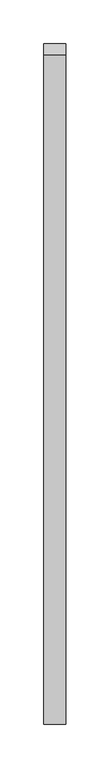
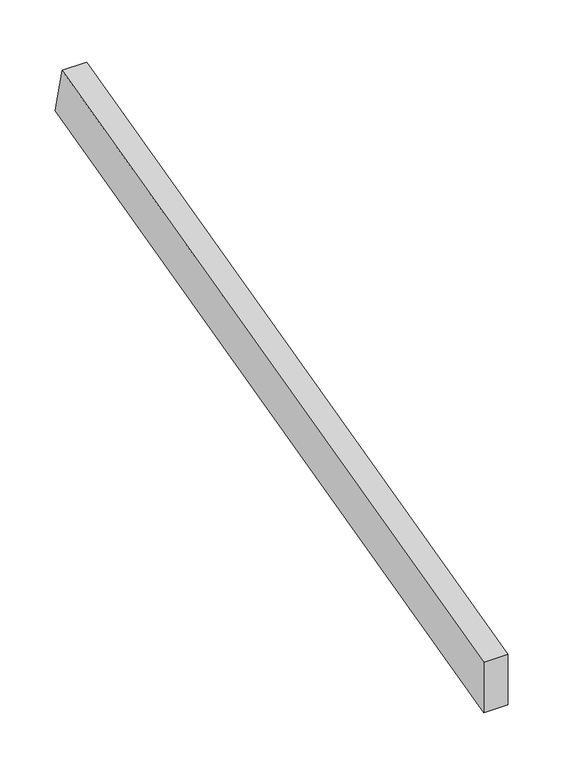
"""IFC4 building model written with IfcOpenShell, lengths in millimetres: proxy geometry, Roof007 1048 : Roof007 1048."""

from ifc_helpers import new_model, si_unit, frame, origin, place, context, project, spatial, polyline, outline, extrude, source, transform, mapped, element, save


def generic_models_48e2aab5(model_context):
    return source(origin(), model_context, "Body", "SweptSolid", [
        extrude(outline(polyline([(8857.5938813, 43486.530071), (9622.975675, 43678.0066467), (9636.2188447, 43625.0339681), (8857.5938813, 43430.3777272), (8857.5938813, 43486.530071)])), frame((5168.9879286, 0.0, 0.0), z_axis=(1.0, 0.0, 0.0), x_axis=(0.0, 1.0, 0.0)), (0.0, 0.0, 1.0), 25.4),
    ])


if __name__ == "__main__":
    model = new_model("IFC4")
    model_context = context("Model", 3, world=origin())
    ifc_project = project(units=[si_unit("LENGTHUNIT", "METRE", prefix="MILLI")], contexts=[model_context])
    site = spatial("IfcSite", under=ifc_project)
    building = spatial("IfcBuilding", under=site)
    placement = place(None, origin())
    generic_models_shape = generic_models_48e2aab5(model_context)
    element("IfcBuildingElementProxy", 1, Name="Roof007 1048 : Roof007 1048", ObjectType="Roof007 1048 : Roof007 1048", at=placement, inside=building, context=model_context, shape_type="MappedRepresentation", body=[
        mapped(generic_models_shape, transform((0.0, 0.0, 0.0), x_axis=(1.0, 0.0, 0.0), y_axis=(0.0, 1.0, 0.0), z_axis=(0.0, 0.0, 1.0))),
    ])
    save(model, "model.ifc")

# Revit data of these elements
# Type "Roof007 1048 : Roof007 1048"
#   NameOverride = "Roof007"
# Element 1 (IfcBuildingElementProxy, "Roof007 1048 : Roof007 1048")
#   Materials on its faces: "STANDING SEAM METAL ROOF"
# Materials
#   "STANDING SEAM METAL ROOF": class "Unassigned", colour RGB 128 128 128, transparency 0
